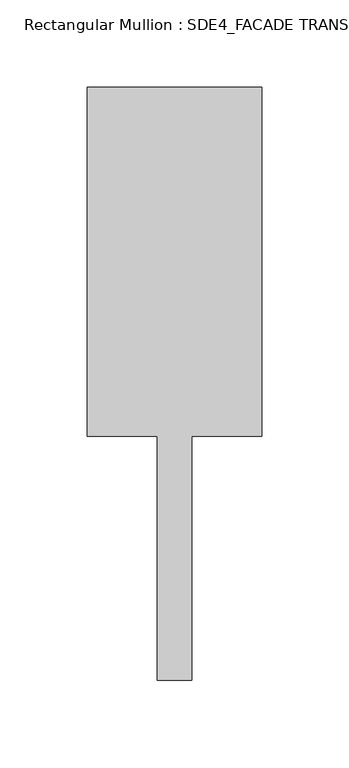
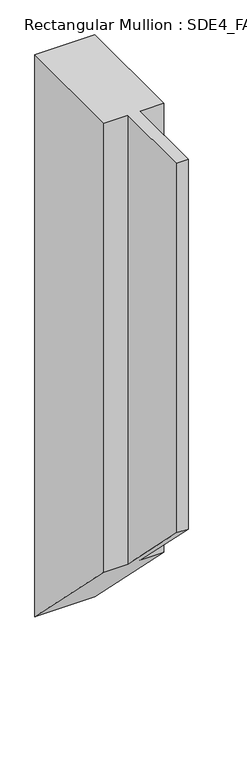
"""IFC4 building model written with IfcOpenShell, lengths in millimetres: member geometry, Rectangular Mullion : SDE4_FACADE TRANSOM TYPE 1."""

from ifc_helpers import new_model, si_unit, origin, place, context, project, spatial, faceted_brep, source, transform, mapped, element, save


def rectangular_mullion_sde4_facade_transom_type_1_20af8dc2(model_context):
    return source(origin(), model_context, "Body", "Brep", [
        faceted_brep([(50.0, 132.5, 0.0), (-50.0, 132.5, 0.0), (-50.0, -67.5, 0.0), (-10.0, -67.5, 0.0), (-10.0, -207.5, 0.0), (10.0, -207.5, 0.0), (10.0, -67.5, 0.0), (50.0, -67.5, 0.0), (50.0, 132.5, -994.0375289), (-50.0, 132.5, -994.0375289), (-50.0, -67.5, -794.0375289), (-10.0, -67.5, -794.0375289), (-10.0, -207.5, -654.0375289), (10.0, -207.5, -654.0375289), (10.0, -67.5, -794.0375289), (50.0, -67.5, -794.0375289)], [[[0, 1, 2, 3, 4, 5, 6, 7]], [[1, 0, 8, 9]], [[2, 1, 9, 10]], [[3, 2, 10, 11]], [[4, 3, 11, 12]], [[5, 4, 12, 13]], [[6, 5, 13, 14]], [[7, 6, 14, 15]], [[0, 7, 15, 8]], [[8, 15, 14, 13, 12, 11, 10, 9]]]),
    ])


if __name__ == "__main__":
    model = new_model("IFC4")
    model_context = context("Model", 3, world=origin())
    ifc_project = project(units=[si_unit("LENGTHUNIT", "METRE", prefix="MILLI")], contexts=[model_context])
    site = spatial("IfcSite", under=ifc_project)
    building = spatial("IfcBuilding", under=site)
    placement = place(None, origin())
    rectangular_mullion_sde4_facade_transom_type_1_shape = rectangular_mullion_sde4_facade_transom_type_1_20af8dc2(model_context)
    element("IfcMember", 1, ObjectType="Rectangular Mullion : SDE4_FACADE TRANSOM TYPE 1", at=placement, inside=building, context=model_context, shape_type="MappedRepresentation", body=[
        mapped(rectangular_mullion_sde4_facade_transom_type_1_shape, transform((0.0, 0.0, 0.0), x_axis=(1.0, 0.0, 0.0), y_axis=(0.0, 1.0, 0.0), z_axis=(0.0, 0.0, 1.0))),
    ])
    save(model, "model.ifc")

# Revit data of these elements
# Type "Rectangular Mullion : SDE4_FACADE TRANSOM TYPE 1"
#   built-in parameter 1007322 = 1.11549 (stored number, unit not read)
#   built-in parameter 1007321 = 0.164042 (stored number, unit not read)
#   built-in parameter 1007320 = 0.164042 (stored number, unit not read)
